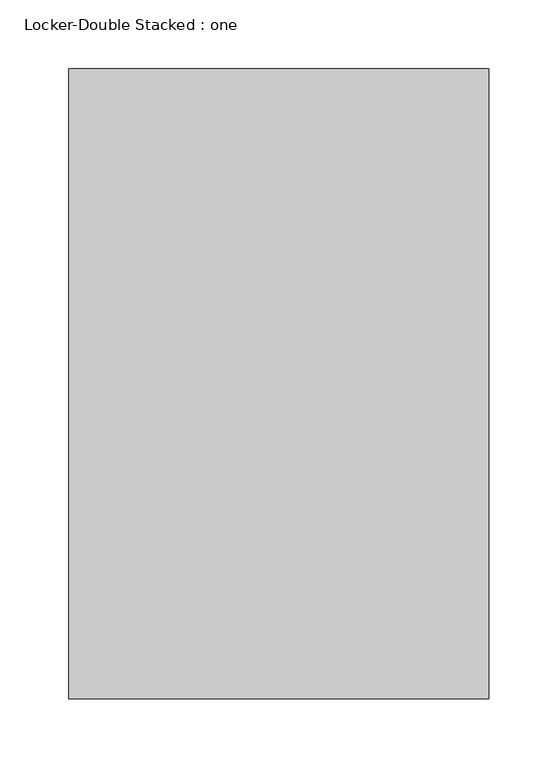
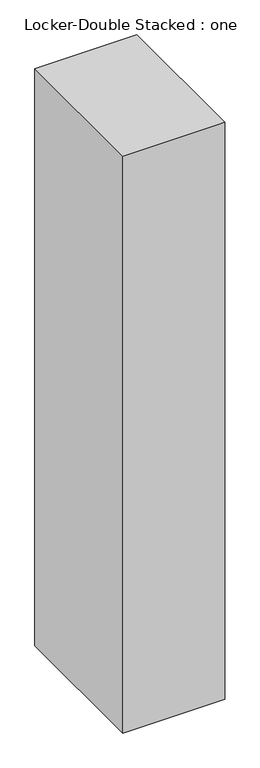
"""IFC4 building model written with IfcOpenShell, lengths in millimetres: furniture geometry, Locker-Double Stacked : one."""

import ifcopenshell
import ifcopenshell.guid

model = None  # the IFC model being written
_history = None  # IfcOwnerHistory: only IFC2X3 demands one
_inside = {}  # id of a spatial element -> (the spatial element, [elements in it])
_under = {}  # id of a project, library or spatial element -> (it, [spatial elements below it])
_declared = {}  # id of a project -> (the project, [libraries it declares])
_typed = {}  # id of a type object -> (the type object, [elements of that type])
_made_of = {}  # id of a material, layer set ... -> (it, [elements and type objects made of it])


def new_model(schema):
    """Start an empty IFC model of exactly this schema.

    Asked for "IFC4X3", IfcOpenShell would pick the latest addendum, in which some entities
    have other attributes; the version numbers below select the first issue.
    IFC2X3 requires an IfcOwnerHistory on every rooted entity: one is made here for all.
    """
    global model, _history
    if schema == "IFC4X3":
        model = ifcopenshell.file(schema_version=(4, 3, 0, 0))
    else:
        model = ifcopenshell.file(schema=schema)
    _inside.clear()
    _under.clear()
    _declared.clear()
    _typed.clear()
    _made_of.clear()
    _history = None
    if model.schema == "IFC2X3":
        org = make("IfcOrganization", Name="unknown")
        user = make(
            "IfcPersonAndOrganization",
            ThePerson=make("IfcPerson", FamilyName="unknown"),
            TheOrganization=org,
        )
        app = make(
            "IfcApplication",
            ApplicationDeveloper=org,
            Version="unknown",
            ApplicationFullName="unknown",
            ApplicationIdentifier="unknown",
        )
        _history = make(
            "IfcOwnerHistory",
            OwningUser=user,
            OwningApplication=app,
            ChangeAction="ADDED",
            CreationDate=0,
        )
    return model


def make(cls, **values):
    """One entity of the class cls with the attributes given. An attribute that is None is left unset."""
    return model.create_entity(
        cls, **{name: value for name, value in values.items() if value is not None}
    )


def rooted(cls, **values):
    """An entity with a GlobalId (a new one), such as an element, a storey or a relation."""
    return make(cls, GlobalId=ifcopenshell.guid.new(), OwnerHistory=_history, **values)


def si_unit(unit_type, name, prefix=None):
    """IfcSIUnit, for example si_unit("LENGTHUNIT", "METRE", prefix="MILLI")."""
    return make("IfcSIUnit", UnitType=unit_type, Prefix=prefix, Name=name)


def assignment(units):
    """IfcUnitAssignment: the units of a project."""
    return None if units is None else make("IfcUnitAssignment", Units=units)


def point(xyz):
    """IfcCartesianPoint."""
    return None if xyz is None else make("IfcCartesianPoint", Coordinates=xyz)


def direction(xyz):
    """IfcDirection."""
    return None if xyz is None else make("IfcDirection", DirectionRatios=xyz)


def frame(location, z_axis=None, x_axis=None):
    """IfcAxis2Placement3D, a coordinate frame: its origin and axes. An axis left out is left unset."""
    return make(
        "IfcAxis2Placement3D",
        Location=point(location),
        Axis=direction(z_axis),
        RefDirection=direction(x_axis),
    )


def origin():
    """The frame at (0, 0, 0) with its axes left unset."""
    return frame((0.0, 0.0, 0.0))


def place(relative_to, where):
    """IfcLocalPlacement: puts the frame where relative to a parent placement (None: the world)."""
    return make(
        "IfcLocalPlacement", PlacementRelTo=relative_to, RelativePlacement=where
    )


def context(
    kind, dimensions, precision=None, world=None, true_north=None, identifier=None
):
    """IfcGeometricRepresentationContext, for example the 3D "Model" context."""
    return make(
        "IfcGeometricRepresentationContext",
        ContextIdentifier=identifier,
        ContextType=kind,
        CoordinateSpaceDimension=dimensions,
        Precision=precision,
        WorldCoordinateSystem=world,
        TrueNorth=true_north,
    )


def project(units=None, contexts=None):
    """IfcProject with its units and contexts."""
    return rooted(
        "IfcProject",
        Name="project",
        RepresentationContexts=contexts,
        UnitsInContext=assignment(units),
    )


def spatial(cls, under=None, at=None, **own):
    """A site, building, storey or space (cls), placed at a placement, below another one or the project."""
    s = rooted(cls, ObjectPlacement=at, **own)
    if under is not None:
        _under.setdefault(under.id(), (under, []))[1].append(s)
    return s


def faces_of(points, faces, orient=None, outer=None):
    """IfcFace entities. A face is a list of loops; a loop is a list of indices into points, from 0.

    orient and outer hold one flag for each loop. By default every Orientation is true, the
    first loop of a face is its IfcFaceOuterBound and the others are IfcFaceBound.
    """
    made = []
    for i, loops in enumerate(faces):
        bounds = []
        for j, loop in enumerate(loops):
            is_outer = j == 0 if outer is None else outer[i][j]
            bounds.append(
                make(
                    "IfcFaceOuterBound" if is_outer else "IfcFaceBound",
                    Bound=make("IfcPolyLoop", Polygon=[points[k] for k in loop]),
                    Orientation=True if orient is None else orient[i][j],
                )
            )
        made.append(make("IfcFace", Bounds=bounds))
    return made


def faceted_brep(points, faces, orient=None, outer=None, voids=None):
    """IfcFacetedBrep: a solid bounded by flat faces; with voids (closed shells), ...WithVoids."""
    shared = [point(p) for p in points]
    hull = make("IfcClosedShell", CfsFaces=faces_of(shared, faces, orient, outer))
    if voids is None:
        return make("IfcFacetedBrep", Outer=hull)
    return make(
        "IfcFacetedBrepWithVoids",
        Outer=hull,
        Voids=[
            make(cls, CfsFaces=faces_of(shared, fs, o, b)) for cls, fs, o, b in voids
        ],
    )


def shape(context_of_items, identifier, shape_type, items):
    """IfcShapeRepresentation: the items that make up one representation, for example the "Body"."""
    return make(
        "IfcShapeRepresentation",
        ContextOfItems=context_of_items,
        RepresentationIdentifier=identifier,
        RepresentationType=shape_type,
        Items=items,
    )


def source(mapping_origin, context_of_items, identifier, shape_type, items):
    """IfcRepresentationMap: a shape defined once, which mapped items show again and again."""
    return make(
        "IfcRepresentationMap",
        MappingOrigin=mapping_origin,
        MappedRepresentation=shape(context_of_items, identifier, shape_type, items),
    )


def transform(
    local_origin,
    x_axis=None,
    y_axis=None,
    z_axis=None,
    scale=None,
    scale2=None,
    scale3=None,
    uniform=True,
):
    """IfcCartesianTransformationOperator3D, or its non-uniform kind. x_axis, y_axis, z_axis: its Axis1, 2, 3."""
    if uniform:
        return make(
            "IfcCartesianTransformationOperator3D",
            Axis1=direction(x_axis),
            Axis2=direction(y_axis),
            LocalOrigin=point(local_origin),
            Scale=scale,
            Axis3=direction(z_axis),
        )
    return make(
        "IfcCartesianTransformationOperator3DnonUniform",
        Axis1=direction(x_axis),
        Axis2=direction(y_axis),
        LocalOrigin=point(local_origin),
        Scale=scale,
        Axis3=direction(z_axis),
        Scale2=scale2,
        Scale3=scale3,
    )


def mapped(mapping_source, mapping_target):
    """IfcMappedItem: shows the shape of a source again, moved by a transform."""
    return make(
        "IfcMappedItem", MappingSource=mapping_source, MappingTarget=mapping_target
    )


def made_of(thing, what):
    """Note that an element or type object is made of a material, layer set ...; save() writes the relation."""
    if what is not None:
        _made_of.setdefault(what.id(), (what, []))[1].append(thing)
    return thing


def element(
    cls,
    number,
    at=None,
    inside=None,
    cuts=None,
    type_object=None,
    material=None,
    context=None,
    identifier="Body",
    shape_type=None,
    held_by="IfcProductDefinitionShape",
    body=None,
    shapes=None,
    **own,
):
    """One element of the class cls, such as IfcWall. Its Tag is "e" and its number.

    at: its placement. inside: the storey or other place that contains it. cuts: it is an
    opening in that element (IfcRelVoidsElement). A single representation is given by context,
    identifier, shape_type and body (its items); several are given by shapes. held_by: the class
    of the entity that holds the representations. save() writes the other relations.
    """
    e = rooted(cls, Tag="e%d" % number, ObjectPlacement=at, **own)
    if body is not None:
        shapes = [shape(context, identifier, shape_type, body)]
    if shapes is not None:
        e.Representation = make(held_by, Representations=shapes)
    if inside is not None:
        _inside.setdefault(inside.id(), (inside, []))[1].append(e)
    if cuts is not None:
        rooted(
            "IfcRelVoidsElement", RelatingBuildingElement=cuts, RelatedOpeningElement=e
        )
    if type_object is not None:
        _typed.setdefault(type_object.id(), (type_object, []))[1].append(e)
    return made_of(e, material)


def aggregate(whole, parts):
    """IfcRelAggregates: a whole, such as a stair, and the parts it consists of."""
    return rooted("IfcRelAggregates", RelatingObject=whole, RelatedObjects=parts)


def save(model, path):
    """Write the relations noted so far, then the file.

    IfcRelAggregates (storeys below a building ...), IfcRelContainedInSpatialStructure (elements
    in a storey), IfcRelDefinesByType, IfcRelAssociatesMaterial and IfcRelDeclares: one each for
    every whole, place, type object, material and project.
    """
    for whole, parts in _under.values():
        aggregate(whole, parts)
    for where, things in _inside.values():
        rooted(
            "IfcRelContainedInSpatialStructure",
            RelatedElements=things,
            RelatingStructure=where,
        )
    for kind, things in _typed.values():
        rooted("IfcRelDefinesByType", RelatedObjects=things, RelatingType=kind)
    for what, things in _made_of.values():
        rooted("IfcRelAssociatesMaterial", RelatedObjects=things, RelatingMaterial=what)
    for by, libraries in _declared.values():
        rooted("IfcRelDeclares", RelatingContext=by, RelatedDefinitions=libraries)
    model.write(path)


def locker_double_stacked_one_7b1cf9e5(model_context):
    return source(origin(), model_context, "Body", "Brep", [
        faceted_brep([(152.4, 228.6, 1828.8), (-152.4, 228.6, 1828.8), (-152.4, -228.6, 1828.8), (152.4, -228.6, 1828.8), (152.4, 228.6, 0.0), (152.4, -228.6, 0.0), (-152.4, -228.6, 0.0), (-152.4, 228.6, 0.0), (127.0, 228.6, 889.0), (-127.0, 228.6, 889.0), (-127.0, 228.6, 76.2), (127.0, 228.6, 76.2), (-127.0, 228.6, 1752.6), (-127.0, 228.6, 939.8), (127.0, 228.6, 939.8), (127.0, 228.6, 1752.6), (127.0, 222.25, 76.2), (-127.0, 222.25, 76.2), (-127.0, 222.25, 889.0), (127.0, 222.25, 889.0), (127.0, 222.25, 1752.6), (127.0, 222.25, 939.8), (-127.0, 222.25, 939.8), (-127.0, 222.25, 1752.6)], [[[0, 1, 2, 3]], [[4, 5, 6, 7]], [[3, 5, 4, 0]], [[2, 6, 5, 3]], [[1, 7, 6, 2]], [[0, 4, 7, 1], [8, 9, 10, 11], [12, 13, 14, 15]], [[16, 17, 18, 19]], [[19, 8, 11, 16]], [[18, 9, 8, 19]], [[17, 10, 9, 18]], [[16, 11, 10, 17]], [[20, 21, 22, 23]], [[23, 12, 15, 20]], [[22, 13, 12, 23]], [[21, 14, 13, 22]], [[20, 15, 14, 21]]]),
    ])


if __name__ == "__main__":
    model = new_model("IFC4")
    model_context = context("Model", 3, world=origin())
    ifc_project = project(units=[si_unit("LENGTHUNIT", "METRE", prefix="MILLI")], contexts=[model_context])
    site = spatial("IfcSite", under=ifc_project)
    building = spatial("IfcBuilding", under=site)
    placement = place(None, origin())
    locker_double_stacked_one_shape = locker_double_stacked_one_7b1cf9e5(model_context)
    element("IfcFurniture", 1, ObjectType="Locker-Double Stacked : one", at=placement, inside=building, context=model_context, shape_type="MappedRepresentation", body=[
        mapped(locker_double_stacked_one_shape, transform((0.0, 0.0, 0.0), x_axis=(1.0, 0.0, 0.0), y_axis=(0.0, 1.0, 0.0), z_axis=(0.0, 0.0, 1.0))),
    ])
    save(model, "model.ifc")

# Revit data of these elements
# Project information
#   Project Issue Date = "07/20/2015"
#   Project Status = "Project Status"
#   Client Name = "Xcel"
#   Project Address = "Enter address here"
#   Project Name = "Xcel Sports Complex - Jefferson, WI"
#   Project Number = "Project Number"
# Type "Locker-Double Stacked : one"
#   Keynote = "M10511300.01"
#   Assembly Code = "E2010"
#   Depth = 1' - 6"
#   Height = 6' - 0"
#   Width = 1' - 0"
#   Material = Metal - Paint Finish - Dark Gray, Matte
# Element 1 (IfcFurniture, "Locker-Double Stacked : one")
#   Materials on its faces: "Metal - Paint Finish - Dark Gray, Matte"
# Materials
#   "Metal - Paint Finish - Dark Gray, Matte": class "Metal", colour RGB 98 98 98, transparency 0
